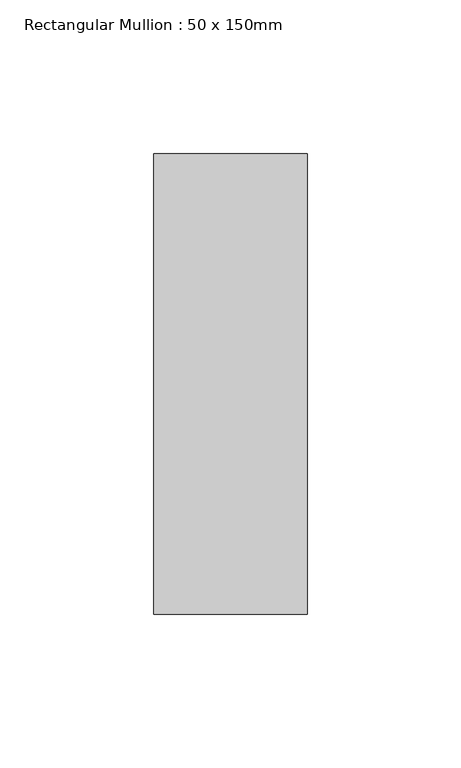
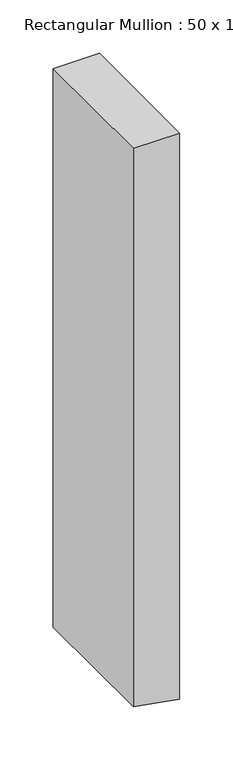
"""IFC4 building model written with IfcOpenShell, lengths in millimetres: member geometry, Rectangular Mullion : 50 x 150mm."""

from ifc_helpers import new_model, si_unit, frame, origin, place, context, project, spatial, polyline, outline, extrude, source, transform, mapped, element, save


def rectangular_mullion_50_x_150mm_226fb8ff(model_context):
    return source(origin(), model_context, "Body", "SweptSolid", [
        extrude(outline(polyline([(0.0, 25.0), (0.0, -25.0), (-638.0829912, -25.0), (-643.2566372, 4.3412044), (-646.8993403, 25.0), (0.0, 25.0)])), frame((0.0, -75.0, 0.0), z_axis=(0.0, 1.0, 0.0), x_axis=(0.0, 0.0, 1.0)), (0.0, 0.0, 1.0), 150.0),
    ])


if __name__ == "__main__":
    model = new_model("IFC4")
    model_context = context("Model", 3, world=origin())
    ifc_project = project(units=[si_unit("LENGTHUNIT", "METRE", prefix="MILLI")], contexts=[model_context])
    site = spatial("IfcSite", under=ifc_project)
    building = spatial("IfcBuilding", under=site)
    placement = place(None, origin())
    rectangular_mullion_50_x_150mm_shape = rectangular_mullion_50_x_150mm_226fb8ff(model_context)
    element("IfcMember", 1, ObjectType="Rectangular Mullion : 50 x 150mm", at=placement, inside=building, context=model_context, shape_type="MappedRepresentation", body=[
        mapped(rectangular_mullion_50_x_150mm_shape, transform((0.0, 0.0, 0.0), x_axis=(1.0, 0.0, 0.0), y_axis=(0.0, 1.0, 0.0), z_axis=(0.0, 0.0, 1.0))),
    ])
    save(model, "model.ifc")

# Revit data of these elements
# Type "Rectangular Mullion : 50 x 150mm"
#   built-in parameter 1007304 = 0.492126 (stored number, unit not read)
#   built-in parameter 1007301 = 0.082021 (stored number, unit not read)
#   built-in parameter 1007300 = 0.082021 (stored number, unit not read)
# Element 1 (IfcMember, "Rectangular Mullion : 50 x 150mm")
#   Materials on its faces: "Aluminium"
# Materials
#   "Aluminium": class "Metal", colour RGB 247 247 247, transparency 0, Description = "Aluminium 6061", Cost = 0
